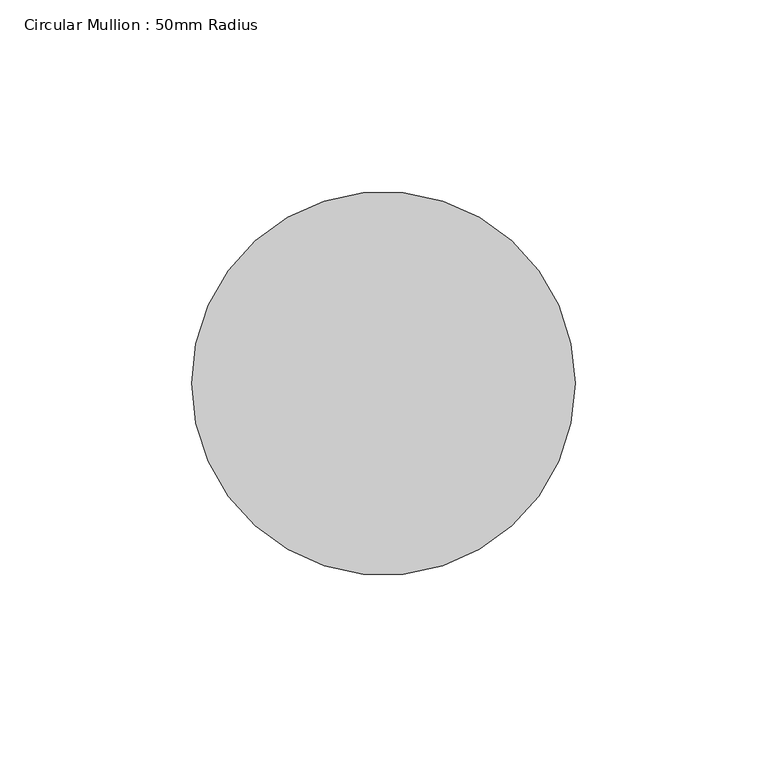
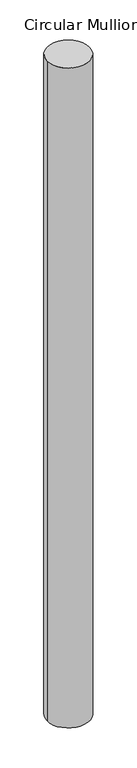
"""IFC4 building model written with IfcOpenShell, lengths in millimetres: member geometry, Circular Mullion : 50mm Radius."""

from ifc_helpers import new_model, si_unit, point, frame, origin, origin_2d, place, context, project, spatial, circle_curve, trimmed, segment, composite_curve, outline, extrude, source, transform, mapped, element, save


def circular_mullion_50mm_radius_717526c0(model_context):
    return source(origin(), model_context, "Body", "SweptSolid", [
        extrude(outline(composite_curve([segment(trimmed(circle_curve(origin_2d(), 50.0), [point((50.0, 0.0))], [point((-50.0, 0.0))], False, "CARTESIAN"), True, "CONTINUOUS"), segment(trimmed(circle_curve(origin_2d(), 50.0), [point((-50.0, 0.0))], [point((50.0, 0.0))], False, "CARTESIAN"), True, "CONTINUOUS")], self_intersect=False)), frame((0.0, 0.0, -1649.4000177), z_axis=(0.0, 0.0, 1.0), x_axis=(1.0, 0.0, 0.0)), (0.0, 0.0, 1.0), 1649.4000177),
    ])


if __name__ == "__main__":
    model = new_model("IFC4")
    model_context = context("Model", 3, world=origin())
    ifc_project = project(units=[si_unit("LENGTHUNIT", "METRE", prefix="MILLI")], contexts=[model_context])
    site = spatial("IfcSite", under=ifc_project)
    building = spatial("IfcBuilding", under=site)
    placement = place(None, origin())
    circular_mullion_50mm_radius_shape = circular_mullion_50mm_radius_717526c0(model_context)
    element("IfcMember", 1, ObjectType="Circular Mullion : 50mm Radius", at=placement, inside=building, context=model_context, shape_type="MappedRepresentation", body=[
        mapped(circular_mullion_50mm_radius_shape, transform((0.0, 0.0, 0.0), x_axis=(1.0, 0.0, 0.0), y_axis=(0.0, 1.0, 0.0), z_axis=(0.0, 0.0, 1.0))),
    ])
    save(model, "model.ifc")

# Revit data of these elements
# Type "Circular Mullion : 50mm Radius"
#   built-in parameter 1007350 = 0.164042 (stored number, unit not read)
# Element 1 (IfcMember, "Circular Mullion : 50mm Radius")
#   Materials on its faces: "Aluminium"
# Materials
#   "Aluminium": class "Metal", colour RGB 247 247 247, transparency 0, Description = "Aluminium 6061", Cost = 0
